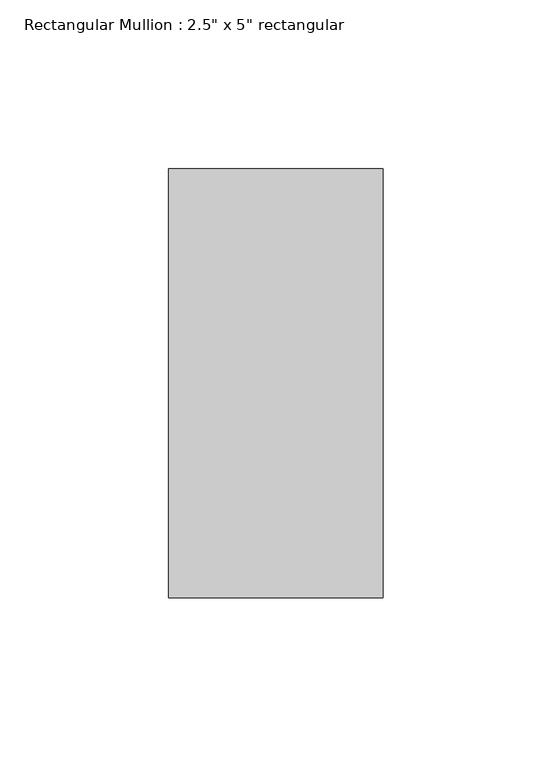
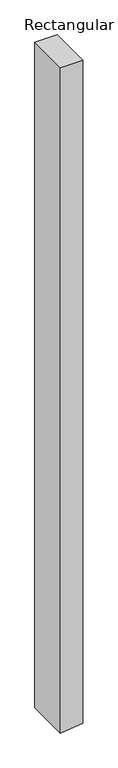
"""IFC4 building model written with IfcOpenShell, lengths in millimetres: member geometry."""

import ifcopenshell
import ifcopenshell.guid

model = None  # the IFC model being written
_history = None  # IfcOwnerHistory: only IFC2X3 demands one
_inside = {}  # id of a spatial element -> (the spatial element, [elements in it])
_under = {}  # id of a project, library or spatial element -> (it, [spatial elements below it])
_declared = {}  # id of a project -> (the project, [libraries it declares])
_typed = {}  # id of a type object -> (the type object, [elements of that type])
_made_of = {}  # id of a material, layer set ... -> (it, [elements and type objects made of it])


def new_model(schema):
    """Start an empty IFC model of exactly this schema.

    Asked for "IFC4X3", IfcOpenShell would pick the latest addendum, in which some entities
    have other attributes; the version numbers below select the first issue.
    IFC2X3 requires an IfcOwnerHistory on every rooted entity: one is made here for all.
    """
    global model, _history
    if schema == "IFC4X3":
        model = ifcopenshell.file(schema_version=(4, 3, 0, 0))
    else:
        model = ifcopenshell.file(schema=schema)
    _inside.clear()
    _under.clear()
    _declared.clear()
    _typed.clear()
    _made_of.clear()
    _history = None
    if model.schema == "IFC2X3":
        org = make("IfcOrganization", Name="unknown")
        user = make(
            "IfcPersonAndOrganization",
            ThePerson=make("IfcPerson", FamilyName="unknown"),
            TheOrganization=org,
        )
        app = make(
            "IfcApplication",
            ApplicationDeveloper=org,
            Version="unknown",
            ApplicationFullName="unknown",
            ApplicationIdentifier="unknown",
        )
        _history = make(
            "IfcOwnerHistory",
            OwningUser=user,
            OwningApplication=app,
            ChangeAction="ADDED",
            CreationDate=0,
        )
    return model


def make(cls, **values):
    """One entity of the class cls with the attributes given. An attribute that is None is left unset."""
    return model.create_entity(
        cls, **{name: value for name, value in values.items() if value is not None}
    )


def rooted(cls, **values):
    """An entity with a GlobalId (a new one), such as an element, a storey or a relation."""
    return make(cls, GlobalId=ifcopenshell.guid.new(), OwnerHistory=_history, **values)


def si_unit(unit_type, name, prefix=None):
    """IfcSIUnit, for example si_unit("LENGTHUNIT", "METRE", prefix="MILLI")."""
    return make("IfcSIUnit", UnitType=unit_type, Prefix=prefix, Name=name)


def assignment(units):
    """IfcUnitAssignment: the units of a project."""
    return None if units is None else make("IfcUnitAssignment", Units=units)


def point(xyz):
    """IfcCartesianPoint."""
    return None if xyz is None else make("IfcCartesianPoint", Coordinates=xyz)


def direction(xyz):
    """IfcDirection."""
    return None if xyz is None else make("IfcDirection", DirectionRatios=xyz)


def frame(location, z_axis=None, x_axis=None):
    """IfcAxis2Placement3D, a coordinate frame: its origin and axes. An axis left out is left unset."""
    return make(
        "IfcAxis2Placement3D",
        Location=point(location),
        Axis=direction(z_axis),
        RefDirection=direction(x_axis),
    )


def origin():
    """The frame at (0, 0, 0) with its axes left unset."""
    return frame((0.0, 0.0, 0.0))


def place(relative_to, where):
    """IfcLocalPlacement: puts the frame where relative to a parent placement (None: the world)."""
    return make(
        "IfcLocalPlacement", PlacementRelTo=relative_to, RelativePlacement=where
    )


def context(
    kind, dimensions, precision=None, world=None, true_north=None, identifier=None
):
    """IfcGeometricRepresentationContext, for example the 3D "Model" context."""
    return make(
        "IfcGeometricRepresentationContext",
        ContextIdentifier=identifier,
        ContextType=kind,
        CoordinateSpaceDimension=dimensions,
        Precision=precision,
        WorldCoordinateSystem=world,
        TrueNorth=true_north,
    )


def project(units=None, contexts=None):
    """IfcProject with its units and contexts."""
    return rooted(
        "IfcProject",
        Name="project",
        RepresentationContexts=contexts,
        UnitsInContext=assignment(units),
    )


def spatial(cls, under=None, at=None, **own):
    """A site, building, storey or space (cls), placed at a placement, below another one or the project."""
    s = rooted(cls, ObjectPlacement=at, **own)
    if under is not None:
        _under.setdefault(under.id(), (under, []))[1].append(s)
    return s


def polyline(points):
    """IfcPolyline through the points."""
    return make("IfcPolyline", Points=[point(p) for p in points])


def outline(outer, holes=None, kind="AREA"):
    """IfcArbitraryClosedProfileDef: a profile drawn as a closed curve; with holes, ...WithVoids."""
    if holes is None:
        return make("IfcArbitraryClosedProfileDef", ProfileType=kind, OuterCurve=outer)
    return make(
        "IfcArbitraryProfileDefWithVoids",
        ProfileType=kind,
        OuterCurve=outer,
        InnerCurves=holes,
    )


def extrude(swept, where, along, depth):
    """IfcExtrudedAreaSolid: the profile swept, set in the frame where, extruded along a direction by depth."""
    return make(
        "IfcExtrudedAreaSolid",
        SweptArea=swept,
        Position=where,
        ExtrudedDirection=direction(along),
        Depth=depth,
    )


def shape(context_of_items, identifier, shape_type, items):
    """IfcShapeRepresentation: the items that make up one representation, for example the "Body"."""
    return make(
        "IfcShapeRepresentation",
        ContextOfItems=context_of_items,
        RepresentationIdentifier=identifier,
        RepresentationType=shape_type,
        Items=items,
    )


def source(mapping_origin, context_of_items, identifier, shape_type, items):
    """IfcRepresentationMap: a shape defined once, which mapped items show again and again."""
    return make(
        "IfcRepresentationMap",
        MappingOrigin=mapping_origin,
        MappedRepresentation=shape(context_of_items, identifier, shape_type, items),
    )


def transform(
    local_origin,
    x_axis=None,
    y_axis=None,
    z_axis=None,
    scale=None,
    scale2=None,
    scale3=None,
    uniform=True,
):
    """IfcCartesianTransformationOperator3D, or its non-uniform kind. x_axis, y_axis, z_axis: its Axis1, 2, 3."""
    if uniform:
        return make(
            "IfcCartesianTransformationOperator3D",
            Axis1=direction(x_axis),
            Axis2=direction(y_axis),
            LocalOrigin=point(local_origin),
            Scale=scale,
            Axis3=direction(z_axis),
        )
    return make(
        "IfcCartesianTransformationOperator3DnonUniform",
        Axis1=direction(x_axis),
        Axis2=direction(y_axis),
        LocalOrigin=point(local_origin),
        Scale=scale,
        Axis3=direction(z_axis),
        Scale2=scale2,
        Scale3=scale3,
    )


def mapped(mapping_source, mapping_target):
    """IfcMappedItem: shows the shape of a source again, moved by a transform."""
    return make(
        "IfcMappedItem", MappingSource=mapping_source, MappingTarget=mapping_target
    )


def made_of(thing, what):
    """Note that an element or type object is made of a material, layer set ...; save() writes the relation."""
    if what is not None:
        _made_of.setdefault(what.id(), (what, []))[1].append(thing)
    return thing


def element(
    cls,
    number,
    at=None,
    inside=None,
    cuts=None,
    type_object=None,
    material=None,
    context=None,
    identifier="Body",
    shape_type=None,
    held_by="IfcProductDefinitionShape",
    body=None,
    shapes=None,
    **own,
):
    """One element of the class cls, such as IfcWall. Its Tag is "e" and its number.

    at: its placement. inside: the storey or other place that contains it. cuts: it is an
    opening in that element (IfcRelVoidsElement). A single representation is given by context,
    identifier, shape_type and body (its items); several are given by shapes. held_by: the class
    of the entity that holds the representations. save() writes the other relations.
    """
    e = rooted(cls, Tag="e%d" % number, ObjectPlacement=at, **own)
    if body is not None:
        shapes = [shape(context, identifier, shape_type, body)]
    if shapes is not None:
        e.Representation = make(held_by, Representations=shapes)
    if inside is not None:
        _inside.setdefault(inside.id(), (inside, []))[1].append(e)
    if cuts is not None:
        rooted(
            "IfcRelVoidsElement", RelatingBuildingElement=cuts, RelatedOpeningElement=e
        )
    if type_object is not None:
        _typed.setdefault(type_object.id(), (type_object, []))[1].append(e)
    return made_of(e, material)


def aggregate(whole, parts):
    """IfcRelAggregates: a whole, such as a stair, and the parts it consists of."""
    return rooted("IfcRelAggregates", RelatingObject=whole, RelatedObjects=parts)


def save(model, path):
    """Write the relations noted so far, then the file.

    IfcRelAggregates (storeys below a building ...), IfcRelContainedInSpatialStructure (elements
    in a storey), IfcRelDefinesByType, IfcRelAssociatesMaterial and IfcRelDeclares: one each for
    every whole, place, type object, material and project.
    """
    for whole, parts in _under.values():
        aggregate(whole, parts)
    for where, things in _inside.values():
        rooted(
            "IfcRelContainedInSpatialStructure",
            RelatedElements=things,
            RelatingStructure=where,
        )
    for kind, things in _typed.values():
        rooted("IfcRelDefinesByType", RelatedObjects=things, RelatingType=kind)
    for what, things in _made_of.values():
        rooted("IfcRelAssociatesMaterial", RelatedObjects=things, RelatingMaterial=what)
    for by, libraries in _declared.values():
        rooted("IfcRelDeclares", RelatingContext=by, RelatedDefinitions=libraries)
    model.write(path)


def member_18682007(model_context):
    return source(origin(), model_context, "Body", "SweptSolid", [
        extrude(outline(polyline([(0.0, 31.75), (0.0, -31.75), (-2017.506255, -31.75), (-2014.7445386, -7.0583463), (-2010.4038959, 31.75), (0.0, 31.75)])), frame((0.0, -63.5, 0.0), z_axis=(0.0, 1.0, 0.0), x_axis=(0.0, 0.0, 1.0)), (0.0, 0.0, 1.0), 127.0),
    ])


if __name__ == "__main__":
    model = new_model("IFC4")
    model_context = context("Model", 3, world=origin())
    ifc_project = project(units=[si_unit("LENGTHUNIT", "METRE", prefix="MILLI")], contexts=[model_context])
    site = spatial("IfcSite", under=ifc_project)
    building = spatial("IfcBuilding", under=site)
    placement = place(None, origin())
    member_shape = member_18682007(model_context)
    element("IfcMember", 1, ObjectType="Rectangular Mullion : 2.5\" x 5\" rectangular", at=placement, inside=building, context=model_context, shape_type="MappedRepresentation", body=[
        mapped(member_shape, transform((0.0, 0.0, 0.0), x_axis=(1.0, 0.0, 0.0), y_axis=(0.0, 1.0, 0.0), z_axis=(0.0, 0.0, 1.0))),
    ])
    save(model, "model.ifc")

# Revit data of these elements
# Type "Rectangular Mullion : 2.5\" x 5\" rectangular"
#   built-in parameter 1007304 = 0.416667 (stored number, unit not read)
#   built-in parameter 1007301 = 0.104167 (stored number, unit not read)
#   built-in parameter 1007300 = 0.104167 (stored number, unit not read)
# Element 1 (IfcMember, "Rectangular Mullion : 2.5\" x 5\" rectangular")
#   Materials on its faces: "Aluminum"
# Materials
#   "Aluminum": class "Metal", colour RGB 247 247 247, transparency 0, Description = "Aluminum 6061", Cost = 0
